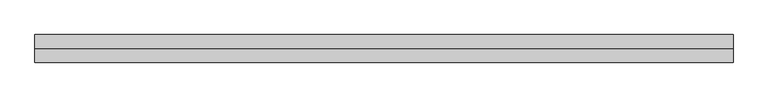
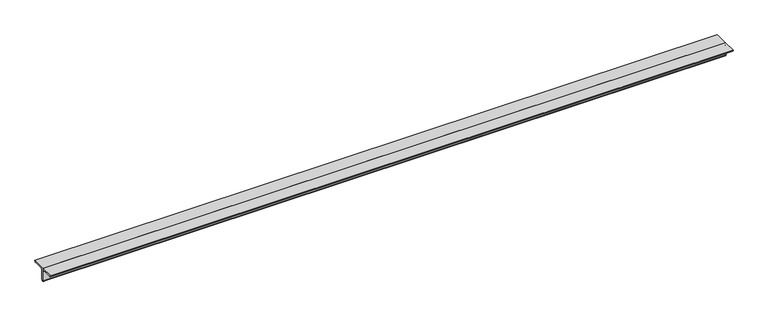
"""IFC4 building model written with IfcOpenShell, lengths in millimetres: member geometry, 0123_Steel Framing_2Ls-KSD3502 : H_SB_AR_S04_2Ls-130x130x12_VBR1."""

from ifc_helpers import new_model, si_unit, point, frame, frame_2d, origin, place, context, project, spatial, polyline, circle_curve, trimmed, segment, composite_curve, outline, extrude, source, transform, mapped, element, save


def member_58c1f9d3(model_context):
    return source(origin(), model_context, "Body", "SweptSolid", [
        extrude(outline(composite_curve([segment(polyline([(0.0, 36.4), (130.0, 36.4)]), True, "CONTINUOUS"), segment(trimmed(circle_curve(frame_2d((118.0, 36.4)), 12.0), [point((130.0, 36.4))], [point((118.0, 24.4))], False, "CARTESIAN"), True, "CONTINUOUS"), segment(polyline([(118.0, 24.4), (24.0, 24.4)]), True, "CONTINUOUS"), segment(trimmed(circle_curve(frame_2d((24.0, 12.4)), 12.0), [point((24.0, 24.4))], [point((12.0, 12.4))], True, "CARTESIAN"), True, "CONTINUOUS"), segment(polyline([(12.0, 12.4), (12.0, -81.6)]), True, "CONTINUOUS"), segment(trimmed(circle_curve(frame_2d((0.0, -81.6)), 12.0), [point((12.0, -81.6))], [point((0.0, -93.6))], False, "CARTESIAN"), True, "CONTINUOUS"), segment(polyline([(0.0, -93.6), (0.0, 36.4)]), True, "CONTINUOUS")], self_intersect=False)), frame((-3283.9548965, 0.0, 0.0), z_axis=(1.0, 0.0, 0.0), x_axis=(0.0, 1.0, 0.0)), (0.0, 0.0, 1.0), 6570.1314861),
        extrude(outline(composite_curve([segment(polyline([(0.0, 36.4), (0.0, -93.6)]), True, "CONTINUOUS"), segment(trimmed(circle_curve(frame_2d((0.0, -81.6)), 12.0), [point((0.0, -93.6))], [point((-12.0, -81.6))], False, "CARTESIAN"), True, "CONTINUOUS"), segment(polyline([(-12.0, -81.6), (-12.0, 12.4)]), True, "CONTINUOUS"), segment(trimmed(circle_curve(frame_2d((-24.0, 12.4)), 12.0), [point((-12.0, 12.4))], [point((-24.0, 24.4))], True, "CARTESIAN"), True, "CONTINUOUS"), segment(polyline([(-24.0, 24.4), (-118.0, 24.4)]), True, "CONTINUOUS"), segment(trimmed(circle_curve(frame_2d((-118.0, 36.4)), 12.0), [point((-118.0, 24.4))], [point((-130.0, 36.4))], False, "CARTESIAN"), True, "CONTINUOUS"), segment(polyline([(-130.0, 36.4), (0.0, 36.4)]), True, "CONTINUOUS")], self_intersect=False)), frame((-3283.9548965, 0.0, 0.0), z_axis=(1.0, 0.0, 0.0), x_axis=(0.0, 1.0, 0.0)), (0.0, 0.0, 1.0), 6570.1314861),
    ])


if __name__ == "__main__":
    model = new_model("IFC4")
    model_context = context("Model", 3, world=origin())
    ifc_project = project(units=[si_unit("LENGTHUNIT", "METRE", prefix="MILLI")], contexts=[model_context])
    site = spatial("IfcSite", under=ifc_project)
    building = spatial("IfcBuilding", under=site)
    placement = place(None, origin())
    member_shape = member_58c1f9d3(model_context)
    element("IfcMember", 1, ObjectType="0123_Steel Framing_2Ls-KSD3502 : H_SB_AR_S04_2Ls-130x130x12_VBR1", at=placement, inside=building, context=model_context, shape_type="MappedRepresentation", body=[
        mapped(member_shape, transform((0.0, 0.0, 0.0), x_axis=(1.0, 0.0, 0.0), y_axis=(0.0, 1.0, 0.0), z_axis=(0.0, 0.0, 1.0))),
    ])
    save(model, "model.ifc")

# Revit data of these elements
# Type "0123_Steel Framing_2Ls-KSD3502 : H_SB_AR_S04_2Ls-130x130x12_VBR1"
#   Assembly Code = "B10"
#   Legs = "SLBB"
#   W = 8.97
#   Perimeter = 1.04 m²/m
#   Nominal Weight = 46.80 kgf/m
#   Length [instance default] = 1000 mm
#   Space = 0 mm
#   b = 130 mm
#   d = 130 mm
#   t = 12 mm
#   y = 36.4 mm
#   A = 0.005952 m²
#   Structural Material [instance default] = Steel ASTM A36
# Element 1 (IfcMember, "0123_Steel Framing_2Ls-KSD3502 : H_SB_AR_S04_2Ls-130x130x12_VBR1")
#   Structural Material = Steel, 45-345
#   Materials on its faces: "Steel, 45-345"
# Materials
#   "Steel ASTM A36": class "Metal", colour RGB 199 199 199, transparency 0, Description = "Structural steel, ASTM A36 Grade B, mill finish", Cost = 0
#   "Steel, 45-345": class "Metal", colour RGB 189 187 185, transparency 0, Description = "Steel 345 MPa", Cost = 0
